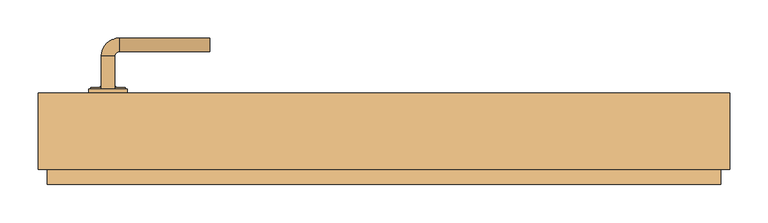
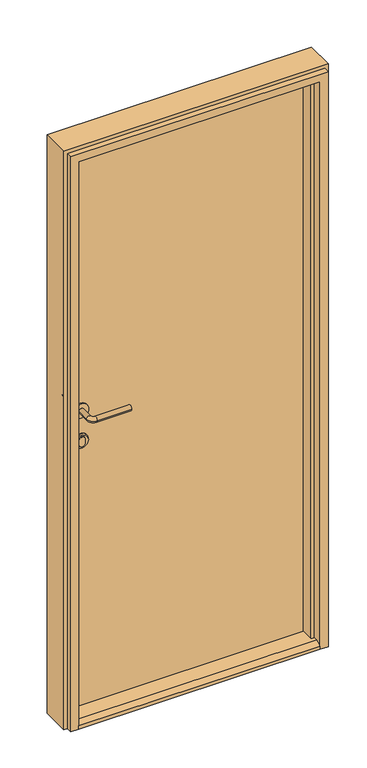
"""IFC4 building model written with IfcOpenShell, lengths in millimetres: door geometry, jeld-wen_interior_door_Stable_GW_single_1.0 : 886 x 2089 mm - M9 x M21."""

import ifcopenshell
import ifcopenshell.guid

model = None  # the IFC model being written
_history = None  # IfcOwnerHistory: only IFC2X3 demands one
_inside = {}  # id of a spatial element -> (the spatial element, [elements in it])
_under = {}  # id of a project, library or spatial element -> (it, [spatial elements below it])
_declared = {}  # id of a project -> (the project, [libraries it declares])
_typed = {}  # id of a type object -> (the type object, [elements of that type])
_made_of = {}  # id of a material, layer set ... -> (it, [elements and type objects made of it])


def new_model(schema):
    """Start an empty IFC model of exactly this schema.

    Asked for "IFC4X3", IfcOpenShell would pick the latest addendum, in which some entities
    have other attributes; the version numbers below select the first issue.
    IFC2X3 requires an IfcOwnerHistory on every rooted entity: one is made here for all.
    """
    global model, _history
    if schema == "IFC4X3":
        model = ifcopenshell.file(schema_version=(4, 3, 0, 0))
    else:
        model = ifcopenshell.file(schema=schema)
    _inside.clear()
    _under.clear()
    _declared.clear()
    _typed.clear()
    _made_of.clear()
    _history = None
    if model.schema == "IFC2X3":
        org = make("IfcOrganization", Name="unknown")
        user = make(
            "IfcPersonAndOrganization",
            ThePerson=make("IfcPerson", FamilyName="unknown"),
            TheOrganization=org,
        )
        app = make(
            "IfcApplication",
            ApplicationDeveloper=org,
            Version="unknown",
            ApplicationFullName="unknown",
            ApplicationIdentifier="unknown",
        )
        _history = make(
            "IfcOwnerHistory",
            OwningUser=user,
            OwningApplication=app,
            ChangeAction="ADDED",
            CreationDate=0,
        )
    return model


def make(cls, **values):
    """One entity of the class cls with the attributes given. An attribute that is None is left unset."""
    return model.create_entity(
        cls, **{name: value for name, value in values.items() if value is not None}
    )


def rooted(cls, **values):
    """An entity with a GlobalId (a new one), such as an element, a storey or a relation."""
    return make(cls, GlobalId=ifcopenshell.guid.new(), OwnerHistory=_history, **values)


def si_unit(unit_type, name, prefix=None):
    """IfcSIUnit, for example si_unit("LENGTHUNIT", "METRE", prefix="MILLI")."""
    return make("IfcSIUnit", UnitType=unit_type, Prefix=prefix, Name=name)


def assignment(units):
    """IfcUnitAssignment: the units of a project."""
    return None if units is None else make("IfcUnitAssignment", Units=units)


def point(xyz):
    """IfcCartesianPoint."""
    return None if xyz is None else make("IfcCartesianPoint", Coordinates=xyz)


def direction(xyz):
    """IfcDirection."""
    return None if xyz is None else make("IfcDirection", DirectionRatios=xyz)


def frame(location, z_axis=None, x_axis=None):
    """IfcAxis2Placement3D, a coordinate frame: its origin and axes. An axis left out is left unset."""
    return make(
        "IfcAxis2Placement3D",
        Location=point(location),
        Axis=direction(z_axis),
        RefDirection=direction(x_axis),
    )


def origin():
    """The frame at (0, 0, 0) with its axes left unset."""
    return frame((0.0, 0.0, 0.0))


def place(relative_to, where):
    """IfcLocalPlacement: puts the frame where relative to a parent placement (None: the world)."""
    return make(
        "IfcLocalPlacement", PlacementRelTo=relative_to, RelativePlacement=where
    )


def context(
    kind, dimensions, precision=None, world=None, true_north=None, identifier=None
):
    """IfcGeometricRepresentationContext, for example the 3D "Model" context."""
    return make(
        "IfcGeometricRepresentationContext",
        ContextIdentifier=identifier,
        ContextType=kind,
        CoordinateSpaceDimension=dimensions,
        Precision=precision,
        WorldCoordinateSystem=world,
        TrueNorth=true_north,
    )


def project(units=None, contexts=None):
    """IfcProject with its units and contexts."""
    return rooted(
        "IfcProject",
        Name="project",
        RepresentationContexts=contexts,
        UnitsInContext=assignment(units),
    )


def spatial(cls, under=None, at=None, **own):
    """A site, building, storey or space (cls), placed at a placement, below another one or the project."""
    s = rooted(cls, ObjectPlacement=at, **own)
    if under is not None:
        _under.setdefault(under.id(), (under, []))[1].append(s)
    return s


def polyline(points):
    """IfcPolyline through the points."""
    return make("IfcPolyline", Points=[point(p) for p in points])


def circle_curve(where, radius):
    """IfcCircle in the frame where."""
    return make("IfcCircle", Position=where, Radius=radius)


def ellipse_curve(where, semi_axis1, semi_axis2):
    """IfcEllipse in the frame where."""
    return make(
        "IfcEllipse", Position=where, SemiAxis1=semi_axis1, SemiAxis2=semi_axis2
    )


def trimmed(basis, trim1, trim2, sense, master):
    """IfcTrimmedCurve: the piece of a basis curve between two trims."""
    return make(
        "IfcTrimmedCurve",
        BasisCurve=basis,
        Trim1=trim1,
        Trim2=trim2,
        SenseAgreement=sense,
        MasterRepresentation=master,
    )


def outline(outer, holes=None, kind="AREA"):
    """IfcArbitraryClosedProfileDef: a profile drawn as a closed curve; with holes, ...WithVoids."""
    if holes is None:
        return make("IfcArbitraryClosedProfileDef", ProfileType=kind, OuterCurve=outer)
    return make(
        "IfcArbitraryProfileDefWithVoids",
        ProfileType=kind,
        OuterCurve=outer,
        InnerCurves=holes,
    )


def extrude(swept, where, along, depth):
    """IfcExtrudedAreaSolid: the profile swept, set in the frame where, extruded along a direction by depth."""
    return make(
        "IfcExtrudedAreaSolid",
        SweptArea=swept,
        Position=where,
        ExtrudedDirection=direction(along),
        Depth=depth,
    )


def faces_of(points, faces, orient=None, outer=None):
    """IfcFace entities. A face is a list of loops; a loop is a list of indices into points, from 0.

    orient and outer hold one flag for each loop. By default every Orientation is true, the
    first loop of a face is its IfcFaceOuterBound and the others are IfcFaceBound.
    """
    made = []
    for i, loops in enumerate(faces):
        bounds = []
        for j, loop in enumerate(loops):
            is_outer = j == 0 if outer is None else outer[i][j]
            bounds.append(
                make(
                    "IfcFaceOuterBound" if is_outer else "IfcFaceBound",
                    Bound=make("IfcPolyLoop", Polygon=[points[k] for k in loop]),
                    Orientation=True if orient is None else orient[i][j],
                )
            )
        made.append(make("IfcFace", Bounds=bounds))
    return made


def faceted_brep(points, faces, orient=None, outer=None, voids=None):
    """IfcFacetedBrep: a solid bounded by flat faces; with voids (closed shells), ...WithVoids."""
    shared = [point(p) for p in points]
    hull = make("IfcClosedShell", CfsFaces=faces_of(shared, faces, orient, outer))
    if voids is None:
        return make("IfcFacetedBrep", Outer=hull)
    return make(
        "IfcFacetedBrepWithVoids",
        Outer=hull,
        Voids=[
            make(cls, CfsFaces=faces_of(shared, fs, o, b)) for cls, fs, o, b in voids
        ],
    )


def shape(context_of_items, identifier, shape_type, items):
    """IfcShapeRepresentation: the items that make up one representation, for example the "Body"."""
    return make(
        "IfcShapeRepresentation",
        ContextOfItems=context_of_items,
        RepresentationIdentifier=identifier,
        RepresentationType=shape_type,
        Items=items,
    )


def source(mapping_origin, context_of_items, identifier, shape_type, items):
    """IfcRepresentationMap: a shape defined once, which mapped items show again and again."""
    return make(
        "IfcRepresentationMap",
        MappingOrigin=mapping_origin,
        MappedRepresentation=shape(context_of_items, identifier, shape_type, items),
    )


def transform(
    local_origin,
    x_axis=None,
    y_axis=None,
    z_axis=None,
    scale=None,
    scale2=None,
    scale3=None,
    uniform=True,
):
    """IfcCartesianTransformationOperator3D, or its non-uniform kind. x_axis, y_axis, z_axis: its Axis1, 2, 3."""
    if uniform:
        return make(
            "IfcCartesianTransformationOperator3D",
            Axis1=direction(x_axis),
            Axis2=direction(y_axis),
            LocalOrigin=point(local_origin),
            Scale=scale,
            Axis3=direction(z_axis),
        )
    return make(
        "IfcCartesianTransformationOperator3DnonUniform",
        Axis1=direction(x_axis),
        Axis2=direction(y_axis),
        LocalOrigin=point(local_origin),
        Scale=scale,
        Axis3=direction(z_axis),
        Scale2=scale2,
        Scale3=scale3,
    )


def mapped(mapping_source, mapping_target):
    """IfcMappedItem: shows the shape of a source again, moved by a transform."""
    return make(
        "IfcMappedItem", MappingSource=mapping_source, MappingTarget=mapping_target
    )


def made_of(thing, what):
    """Note that an element or type object is made of a material, layer set ...; save() writes the relation."""
    if what is not None:
        _made_of.setdefault(what.id(), (what, []))[1].append(thing)
    return thing


def element(
    cls,
    number,
    at=None,
    inside=None,
    cuts=None,
    type_object=None,
    material=None,
    context=None,
    identifier="Body",
    shape_type=None,
    held_by="IfcProductDefinitionShape",
    body=None,
    shapes=None,
    **own,
):
    """One element of the class cls, such as IfcWall. Its Tag is "e" and its number.

    at: its placement. inside: the storey or other place that contains it. cuts: it is an
    opening in that element (IfcRelVoidsElement). A single representation is given by context,
    identifier, shape_type and body (its items); several are given by shapes. held_by: the class
    of the entity that holds the representations. save() writes the other relations.
    """
    e = rooted(cls, Tag="e%d" % number, ObjectPlacement=at, **own)
    if body is not None:
        shapes = [shape(context, identifier, shape_type, body)]
    if shapes is not None:
        e.Representation = make(held_by, Representations=shapes)
    if inside is not None:
        _inside.setdefault(inside.id(), (inside, []))[1].append(e)
    if cuts is not None:
        rooted(
            "IfcRelVoidsElement", RelatingBuildingElement=cuts, RelatedOpeningElement=e
        )
    if type_object is not None:
        _typed.setdefault(type_object.id(), (type_object, []))[1].append(e)
    return made_of(e, material)


def aggregate(whole, parts):
    """IfcRelAggregates: a whole, such as a stair, and the parts it consists of."""
    return rooted("IfcRelAggregates", RelatingObject=whole, RelatedObjects=parts)


def save(model, path):
    """Write the relations noted so far, then the file.

    IfcRelAggregates (storeys below a building ...), IfcRelContainedInSpatialStructure (elements
    in a storey), IfcRelDefinesByType, IfcRelAssociatesMaterial and IfcRelDeclares: one each for
    every whole, place, type object, material and project.
    """
    for whole, parts in _under.values():
        aggregate(whole, parts)
    for where, things in _inside.values():
        rooted(
            "IfcRelContainedInSpatialStructure",
            RelatedElements=things,
            RelatingStructure=where,
        )
    for kind, things in _typed.values():
        rooted("IfcRelDefinesByType", RelatedObjects=things, RelatingType=kind)
    for what, things in _made_of.values():
        rooted("IfcRelAssociatesMaterial", RelatedObjects=things, RelatingMaterial=what)
    for by, libraries in _declared.values():
        rooted("IfcRelDeclares", RelatingContext=by, RelatedDefinitions=libraries)
    model.write(path)


def plane_surface(at):
    """IfcPlane: the flat surface through the origin of the frame at, square to its z axis."""
    return make("IfcPlane", Position=at)


def cylinder_surface(at, radius):
    """IfcCylindricalSurface: all points at the distance radius from the z axis of the frame at."""
    return make("IfcCylindricalSurface", Position=at, Radius=radius)


def revolved_surface(curve, axis_point, axis_direction):
    """IfcSurfaceOfRevolution: the curve turned about the line through axis_point along axis_direction."""
    return make(
        "IfcSurfaceOfRevolution",
        SweptCurve=make("IfcArbitraryOpenProfileDef", ProfileType="CURVE", Curve=curve),
        AxisPosition=make("IfcAxis1Placement", Location=point(axis_point), Axis=direction(axis_direction)),
    )


def advanced_brep(points, edges, surfaces, faces):
    """IfcAdvancedBrep: a solid bounded by faces that lie on surfaces and meet in shared edges.

    An edge is (start, end): straight between two places in points (the first is 0);
    or (start, end, curve); or (start, end, curve, False) where it runs against its curve.
    A face is (place in surfaces, loops), or (place, loops, False) where it looks against
    its surface's normal. A loop lists edges by number (the first is 1), with a minus sign
    where the edge is run from its end to its start. The first loop is the outer one.
    """
    corners = [point(p) for p in points]
    vertices = [make("IfcVertexPoint", VertexGeometry=c) for c in corners]
    made = []
    for start, end, *more in edges:
        made.append(
            make(
                "IfcEdgeCurve",
                EdgeStart=vertices[start],
                EdgeEnd=vertices[end],
                EdgeGeometry=more[0] if more else make("IfcPolyline", Points=[corners[start], corners[end]]),
                SameSense=more[1] if len(more) > 1 else True,
            )
        )
    hull = []
    for where, loops, *sense in faces:
        bounds = []
        for j, loop in enumerate(loops):
            ring = [make("IfcOrientedEdge", EdgeElement=made[abs(k) - 1], Orientation=k > 0) for k in loop]
            bounds.append(
                make(
                    "IfcFaceOuterBound" if j == 0 else "IfcFaceBound",
                    Bound=make("IfcEdgeLoop", EdgeList=ring),
                    Orientation=True,
                )
            )
        hull.append(make("IfcAdvancedFace", Bounds=bounds, FaceSurface=surfaces[where], SameSense=sense[0] if sense else True))
    return make("IfcAdvancedBrep", Outer=make("IfcClosedShell", CfsFaces=hull))


def door_ee319b5f(model_context):
    return source(origin(), model_context, "Body", "SolidModel", [
        advanced_brep(
        [(-385.4704625, 2.0, 983.0), (-340.4704625, 2.0, 983.0), (-371.7998782, 2.0, 995.5684608), (-363.4704625, 2.0, 1000.5), (-362.4704625, 2.0, 1000.5), (-352.9704625, 2.0, 991.0), (-352.9704625, 2.0, 975.0), (-362.4704625, 2.0, 965.5), (-363.4704625, 2.0, 965.5), (-372.9704625, 2.0, 975.0), (-372.9704625, 2.0, 991.0), (-387.9704625, 8.0, 983.0), (-337.9704625, 8.0, 983.0), (-387.9704625, 10.0, 983.0), (-337.9704625, 10.0, 983.0), (-363.4704625, 1.0, 1000.5), (-371.7998782, 1.0, 995.5684608), (-372.9704625, 1.0, 991.0), (-372.9704625, 1.0, 975.0), (-363.4704625, 1.0, 965.5), (-362.4704625, 1.0, 965.5), (-352.9704625, 1.0, 975.0), (-352.9704625, 1.0, 991.0), (-362.4704625, 1.0, 1000.5)],
        [
            (0, 1, circle_curve(frame((-362.9704625, 2.0, 983.0), z_axis=(0.0, -1.0, 0.0), x_axis=(-1.0, 0.0, 0.0)), 22.5)),
            (1, 0, circle_curve(frame((-362.9704625, 2.0, 983.0), z_axis=(0.0, -1.0, 0.0), x_axis=(1.0, 0.0, 0.0)), 22.5)),
            (2, 3, circle_curve(frame((-363.4704625, 2.0, 991.0), z_axis=(0.0, 1.0, 0.0), x_axis=(-1.0, 0.0, 0.0)), 9.5)),
            (3, 4),
            (4, 5, circle_curve(frame((-362.4704625, 2.0, 991.0), z_axis=(0.0, 1.0, 0.0), x_axis=(-1.0, 0.0, 0.0)), 9.5)),
            (5, 6),
            (6, 7, circle_curve(frame((-362.4704625, 2.0, 975.0), z_axis=(0.0, 1.0, 0.0), x_axis=(-1.0, 0.0, 0.0)), 9.5)),
            (7, 8),
            (8, 9, circle_curve(frame((-363.4704625, 2.0, 975.0), z_axis=(0.0, 1.0, 0.0), x_axis=(-1.0, 0.0, 0.0)), 9.5)),
            (9, 10),
            (10, 2, circle_curve(frame((-363.4704625, 2.0, 991.0), z_axis=(0.0, 1.0, 0.0), x_axis=(-1.0, 0.0, 0.0)), 9.5)),
            (0, 11),
            (11, 12, circle_curve(frame((-362.9704625, 8.0, 983.0), z_axis=(0.0, -1.0, 0.0), x_axis=(-1.0, 0.0, 0.0)), 25.0)),
            (12, 1),
            (12, 11, circle_curve(frame((-362.9704625, 8.0, 983.0), z_axis=(0.0, -1.0, 0.0), x_axis=(1.0, 0.0, 0.0)), 25.0)),
            (13, 14, circle_curve(frame((-362.9704625, 10.0, 983.0), z_axis=(0.0, 1.0, 0.0), x_axis=(1.0, 0.0, 0.0)), 25.0)),
            (14, 13, circle_curve(frame((-362.9704625, 10.0, 983.0), z_axis=(0.0, 1.0, 0.0), x_axis=(1.0, 0.0, 0.0)), 25.0)),
            (14, 12),
            (11, 13),
            (15, 16, circle_curve(frame((-363.4704625, 1.0, 991.0), z_axis=(0.0, -1.0, 0.0), x_axis=(-1.0, 0.0, 0.0)), 9.5)),
            (16, 17, circle_curve(frame((-363.4704625, 1.0, 991.0), z_axis=(0.0, -1.0, 0.0), x_axis=(-1.0, 0.0, 0.0)), 9.5)),
            (17, 18),
            (18, 19, circle_curve(frame((-363.4704625, 1.0, 975.0), z_axis=(0.0, -1.0, 0.0), x_axis=(-1.0, 0.0, 0.0)), 9.5)),
            (19, 20),
            (20, 21, circle_curve(frame((-362.4704625, 1.0, 975.0), z_axis=(0.0, -1.0, 0.0), x_axis=(-1.0, 0.0, 0.0)), 9.5)),
            (21, 22),
            (22, 23, circle_curve(frame((-362.4704625, 1.0, 991.0), z_axis=(0.0, -1.0, 0.0), x_axis=(-1.0, 0.0, 0.0)), 9.5)),
            (23, 15),
            (15, 3),
            (2, 16),
            (10, 17),
            (9, 18),
            (8, 19),
            (7, 20),
            (6, 21),
            (5, 22),
            (4, 23),
        ],
        [
            plane_surface(frame((-362.9704625, 2.0, 983.0), z_axis=(0.0, -1.0, 0.0), x_axis=(0.0, 0.0, -1.0))),
            revolved_surface(polyline([(-385.4704625, 2.0, 983.0), (-387.9704625, 8.0, 983.0)]), (-362.9704625, -52.0, 983.0), (0.0, 1.0, 0.0)),
            revolved_surface(polyline([(-340.4704625, 2.0, 983.0), (-337.9704625, 8.0, 983.0)]), (-362.9704625, -52.0, 983.0), (0.0, 1.0, 0.0)),
            plane_surface(frame((-337.9704625, 10.0, 983.0), z_axis=(0.0, 1.0, 0.0), x_axis=(0.0, 0.0, -1.0))),
            cylinder_surface(frame((-362.9704625, 10.0, 983.0), z_axis=(0.0, -1.0, 0.0), x_axis=(1.0, 0.0, 0.0)), 25.0),
            plane_surface(frame((-372.9704625, 1.0, 991.0), z_axis=(0.0, -1.0, 0.0), x_axis=(0.0, 0.0, -1.0))),
            cylinder_surface(frame((-363.4704625, 2.0, 991.0), z_axis=(0.0, -1.0, 0.0), x_axis=(-1.0, 0.0, 0.0)), 9.5),
            plane_surface(frame((-372.9704625, 1.0, 991.0), z_axis=(-1.0, 0.0, 0.0), x_axis=(0.0, 1.0, 0.0))),
            cylinder_surface(frame((-363.4704625, 2.0, 975.0), z_axis=(0.0, -1.0, 0.0), x_axis=(-1.0, 0.0, 0.0)), 9.5),
            plane_surface(frame((-363.4704625, 1.0, 965.5), z_axis=(0.0, 0.0, -1.0), x_axis=(0.0, 1.0, 0.0))),
            cylinder_surface(frame((-362.4704625, 2.0, 975.0), z_axis=(0.0, -1.0, 0.0), x_axis=(-1.0, 0.0, 0.0)), 9.5),
            plane_surface(frame((-352.9704625, 1.0, 975.0), z_axis=(1.0, 0.0, 0.0), x_axis=(0.0, 1.0, 0.0))),
            cylinder_surface(frame((-362.4704625, 2.0, 991.0), z_axis=(0.0, -1.0, 0.0), x_axis=(-1.0, 0.0, 0.0)), 9.5),
            plane_surface(frame((-362.4704625, 1.0, 1000.5), z_axis=(0.0, 0.0, 1.0), x_axis=(0.0, 1.0, 0.0))),
        ],
        [
            (0, [[1, 2], [3, 4, 5, 6, 7, 8, 9, 10, 11]]),
            (1, [[-1, 12, 13, 14]]),
            (2, [[-2, -14, 15, -12]]),
            (3, [[16, 17]]),
            (4, [[-17, 18, -13, 19]]),
            (4, [[-16, -19, -15, -18]]),
            (5, [[20, 21, 22, 23, 24, 25, 26, 27, 28]]),
            (6, [[-20, 29, -3, 30]]),
            (6, [[-21, -30, -11, 31]]),
            (7, [[-22, -31, -10, 32]]),
            (8, [[-23, -32, -9, 33]]),
            (9, [[-24, -33, -8, 34]]),
            (10, [[-25, -34, -7, 35]]),
            (11, [[-26, -35, -6, 36]]),
            (12, [[-27, -36, -5, 37]]),
            (13, [[-28, -37, -4, -29]]),
        ],
    ),
        advanced_brep(
        [(-385.4704625, 58.0, 983.0), (-340.4704625, 58.0, 983.0), (-371.7998782, 58.0, 995.5684608), (-372.9704625, 58.0, 991.0), (-372.9704625, 58.0, 975.0), (-363.4704625, 58.0, 965.5), (-362.4704625, 58.0, 965.5), (-352.9704625, 58.0, 975.0), (-352.9704625, 58.0, 991.0), (-362.4704625, 58.0, 1000.5), (-363.4704625, 58.0, 1000.5), (-337.9704625, 52.0, 983.0), (-387.9704625, 52.0, 983.0), (-387.9704625, 50.0, 983.0), (-337.9704625, 50.0, 983.0), (-363.4704625, 59.0, 1000.5), (-362.4704625, 59.0, 1000.5), (-352.9704625, 59.0, 991.0), (-352.9704625, 59.0, 975.0), (-362.4704625, 59.0, 965.5), (-363.4704625, 59.0, 965.5), (-372.9704625, 59.0, 975.0), (-372.9704625, 59.0, 991.0), (-371.7998782, 59.0, 995.5684608)],
        [
            (0, 1, circle_curve(frame((-362.9704625, 58.0, 983.0), z_axis=(0.0, 1.0, 0.0), x_axis=(1.0, 0.0, 0.0)), 22.5)),
            (1, 0, circle_curve(frame((-362.9704625, 58.0, 983.0), z_axis=(0.0, 1.0, 0.0), x_axis=(-1.0, 0.0, 0.0)), 22.5)),
            (2, 3, circle_curve(frame((-363.4704625, 58.0, 991.0), z_axis=(0.0, -1.0, 0.0), x_axis=(-1.0, 0.0, 0.0)), 9.5)),
            (3, 4),
            (4, 5, circle_curve(frame((-363.4704625, 58.0, 975.0), z_axis=(0.0, -1.0, 0.0), x_axis=(-1.0, 0.0, 0.0)), 9.5)),
            (5, 6),
            (6, 7, circle_curve(frame((-362.4704625, 58.0, 975.0), z_axis=(0.0, -1.0, 0.0), x_axis=(-1.0, 0.0, 0.0)), 9.5)),
            (7, 8),
            (8, 9, circle_curve(frame((-362.4704625, 58.0, 991.0), z_axis=(0.0, -1.0, 0.0), x_axis=(-1.0, 0.0, 0.0)), 9.5)),
            (9, 10),
            (10, 2, circle_curve(frame((-363.4704625, 58.0, 991.0), z_axis=(0.0, -1.0, 0.0), x_axis=(-1.0, 0.0, 0.0)), 9.5)),
            (1, 11),
            (11, 12, circle_curve(frame((-362.9704625, 52.0, 983.0), z_axis=(0.0, 1.0, 0.0), x_axis=(-1.0, 0.0, 0.0)), 25.0)),
            (12, 0),
            (12, 11, circle_curve(frame((-362.9704625, 52.0, 983.0), z_axis=(0.0, 1.0, 0.0), x_axis=(1.0, 0.0, 0.0)), 25.0)),
            (13, 14, circle_curve(frame((-362.9704625, 50.0, 983.0), z_axis=(0.0, -1.0, 0.0), x_axis=(1.0, 0.0, 0.0)), 25.0)),
            (14, 13, circle_curve(frame((-362.9704625, 50.0, 983.0), z_axis=(0.0, -1.0, 0.0), x_axis=(1.0, 0.0, 0.0)), 25.0)),
            (13, 12),
            (11, 14),
            (15, 16),
            (16, 17, circle_curve(frame((-362.4704625, 59.0, 991.0), z_axis=(0.0, 1.0, 0.0), x_axis=(-1.0, 0.0, 0.0)), 9.5)),
            (17, 18),
            (18, 19, circle_curve(frame((-362.4704625, 59.0, 975.0), z_axis=(0.0, 1.0, 0.0), x_axis=(-1.0, 0.0, 0.0)), 9.5)),
            (19, 20),
            (20, 21, circle_curve(frame((-363.4704625, 59.0, 975.0), z_axis=(0.0, 1.0, 0.0), x_axis=(-1.0, 0.0, 0.0)), 9.5)),
            (21, 22),
            (22, 23, circle_curve(frame((-363.4704625, 59.0, 991.0), z_axis=(0.0, 1.0, 0.0), x_axis=(-1.0, 0.0, 0.0)), 9.5)),
            (23, 15, circle_curve(frame((-363.4704625, 59.0, 991.0), z_axis=(0.0, 1.0, 0.0), x_axis=(-1.0, 0.0, 0.0)), 9.5)),
            (23, 2),
            (10, 15),
            (22, 3),
            (21, 4),
            (20, 5),
            (19, 6),
            (18, 7),
            (17, 8),
            (16, 9),
        ],
        [
            plane_surface(frame((-362.9704625, 58.0, 983.0), z_axis=(0.0, 1.0, 0.0), x_axis=(0.0, 0.0, -1.0))),
            revolved_surface(polyline([(-340.4704625, 58.0, 983.0), (-337.9704625, 52.0, 983.0)]), (-362.9704625, 112.0, 983.0), (0.0, -1.0, 0.0)),
            revolved_surface(polyline([(-385.4704625, 58.0, 983.0), (-387.9704625, 52.0, 983.0)]), (-362.9704625, 112.0, 983.0), (0.0, -1.0, 0.0)),
            plane_surface(frame((-337.9704625, 50.0, 983.0), z_axis=(0.0, -1.0, 0.0), x_axis=(0.0, 0.0, -1.0))),
            cylinder_surface(frame((-362.9704625, 50.0, 983.0), z_axis=(0.0, 1.0, 0.0), x_axis=(1.0, 0.0, 0.0)), 25.0),
            plane_surface(frame((-372.9704625, 59.0, 991.0), z_axis=(0.0, 1.0, 0.0), x_axis=(0.0, 0.0, -1.0))),
            cylinder_surface(frame((-363.4704625, 58.0, 991.0), z_axis=(0.0, 1.0, 0.0), x_axis=(-1.0, 0.0, 0.0)), 9.5),
            plane_surface(frame((-372.9704625, 59.0, 991.0), z_axis=(-1.0, 0.0, 0.0), x_axis=(0.0, -1.0, 0.0))),
            cylinder_surface(frame((-363.4704625, 58.0, 975.0), z_axis=(0.0, 1.0, 0.0), x_axis=(-1.0, 0.0, 0.0)), 9.5),
            plane_surface(frame((-363.4704625, 59.0, 965.5), z_axis=(0.0, 0.0, -1.0), x_axis=(0.0, -1.0, 0.0))),
            cylinder_surface(frame((-362.4704625, 58.0, 975.0), z_axis=(0.0, 1.0, 0.0), x_axis=(-1.0, 0.0, 0.0)), 9.5),
            plane_surface(frame((-352.9704625, 59.0, 975.0), z_axis=(1.0, 0.0, 0.0), x_axis=(0.0, -1.0, 0.0))),
            cylinder_surface(frame((-362.4704625, 58.0, 991.0), z_axis=(0.0, 1.0, 0.0), x_axis=(-1.0, 0.0, 0.0)), 9.5),
            plane_surface(frame((-362.4704625, 59.0, 1000.5), z_axis=(0.0, 0.0, 1.0), x_axis=(0.0, -1.0, 0.0))),
        ],
        [
            (0, [[1, 2], [3, 4, 5, 6, 7, 8, 9, 10, 11]]),
            (1, [[12, 13, 14, -2]]),
            (2, [[-14, 15, -12, -1]]),
            (3, [[16, 17]]),
            (4, [[18, -13, 19, -16]]),
            (4, [[-19, -15, -18, -17]]),
            (5, [[20, 21, 22, 23, 24, 25, 26, 27, 28]]),
            (6, [[29, -11, 30, -28]]),
            (6, [[31, -3, -29, -27]]),
            (7, [[32, -4, -31, -26]]),
            (8, [[33, -5, -32, -25]]),
            (9, [[34, -6, -33, -24]]),
            (10, [[35, -7, -34, -23]]),
            (11, [[36, -8, -35, -22]]),
            (12, [[37, -9, -36, -21]]),
            (13, [[-30, -10, -37, -20]]),
        ],
    ),
        advanced_brep(
        [(-387.9704625, 4.0, 1093.0), (-337.9704625, 4.0, 1093.0), (-354.0050698, 4.0, 1093.0), (-371.9358552, 4.0, 1093.0), (-387.9704625, 10.0, 1093.0), (-337.9704625, 10.0, 1093.0), (-371.9358552, -38.9627146, 1093.0), (-354.0050698, -38.9627146, 1093.0), (-347.9704625, -62.9281073, 1093.0), (-347.9704625, -44.9973219, 1093.0), (-228.9704625, -44.9973219, 1093.0), (-228.9704625, -62.9281073, 1093.0)],
        [
            (0, 1, circle_curve(frame((-362.9704625, 4.0, 1093.0), z_axis=(0.0, -1.0, 0.0), x_axis=(1.0, 0.0, 0.0)), 25.0)),
            (1, 0, circle_curve(frame((-362.9704625, 4.0, 1093.0), z_axis=(0.0, -1.0, 0.0), x_axis=(1.0, 0.0, 0.0)), 25.0)),
            (2, 3, circle_curve(frame((-362.9704625, 4.0, 1093.0), z_axis=(0.0, 1.0, 0.0), x_axis=(-1.0, 0.0, 0.0)), 8.9653927)),
            (3, 2, circle_curve(frame((-362.9704625, 4.0, 1093.0), z_axis=(0.0, 1.0, 0.0), x_axis=(-1.0, 0.0, 0.0)), 8.9653927)),
            (4, 5, circle_curve(frame((-362.9704625, 10.0, 1093.0), z_axis=(0.0, 1.0, 0.0), x_axis=(1.0, 0.0, 0.0)), 25.0)),
            (5, 4, circle_curve(frame((-362.9704625, 10.0, 1093.0), z_axis=(0.0, 1.0, 0.0), x_axis=(1.0, 0.0, 0.0)), 25.0)),
            (0, 4),
            (5, 1),
            (3, 6),
            (6, 7, circle_curve(frame((-362.9704625, -38.9627146, 1093.0), z_axis=(0.0, 1.0, 0.0), x_axis=(-1.0, 0.0, 0.0)), 8.9653927)),
            (7, 2),
            (7, 6, circle_curve(frame((-362.9704625, -38.9627146, 1093.0), z_axis=(0.0, 1.0, 0.0), x_axis=(-1.0, 0.0, 0.0)), 8.9653927)),
            (6, 8, circle_curve(frame((-347.9704625, -38.9627146, 1093.0), z_axis=(0.0, 0.0, 1.0), x_axis=(-1.0, 0.0, 0.0)), 23.9653927)),
            (8, 9, circle_curve(frame((-347.9704625, -53.9627146, 1093.0), z_axis=(-1.0, 0.0, 0.0), x_axis=(0.0, -1.0, 0.0)), 8.9653927)),
            (9, 7, circle_curve(frame((-347.9704625, -38.9627146, 1093.0), z_axis=(0.0, 0.0, -1.0), x_axis=(-1.0, 0.0, 0.0)), 6.0346073)),
            (9, 8, circle_curve(frame((-347.9704625, -53.9627146, 1093.0), z_axis=(-1.0, 0.0, 0.0), x_axis=(0.0, -1.0, 0.0)), 8.9653927)),
            (10, 11, circle_curve(frame((-228.9704625, -53.9627146, 1093.0), z_axis=(1.0, 0.0, 0.0), x_axis=(0.0, -1.0, 0.0)), 8.9653927)),
            (11, 10, circle_curve(frame((-228.9704625, -53.9627146, 1093.0), z_axis=(1.0, 0.0, 0.0), x_axis=(0.0, -1.0, 0.0)), 8.9653927)),
            (8, 11),
            (10, 9),
        ],
        [
            plane_surface(frame((-337.9704625, 4.0, 1093.0), z_axis=(0.0, -1.0, 0.0), x_axis=(0.0, 0.0, -1.0))),
            plane_surface(frame((-337.9704625, 10.0, 1093.0), z_axis=(0.0, 1.0, 0.0), x_axis=(0.0, 0.0, 1.0))),
            cylinder_surface(frame((-362.9704625, 4.0, 1093.0), z_axis=(0.0, 1.0, 0.0), x_axis=(1.0, 0.0, 0.0)), 25.0),
            cylinder_surface(frame((-362.9704625, 4.0, 1093.0), z_axis=(0.0, 1.0, 0.0), x_axis=(-1.0, 0.0, 0.0)), 8.9653927),
            revolved_surface(trimmed(ellipse_curve(frame((-362.9704625, -38.9627146, 1093.0), z_axis=(0.0, -1.0, 0.0), x_axis=(-1.0, 0.0, 0.0)), 8.9653927, 8.9653927), [point((-354.0050698, -38.9627146, 1093.0))], [point((-371.9358552, -38.9627146, 1093.0))], True, "CARTESIAN"), (-347.9704625, -38.9627146, 1093.0), (0.0, 0.0, -1.0)),
            revolved_surface(trimmed(ellipse_curve(frame((-362.9704625, -38.9627146, 1093.0), z_axis=(0.0, -1.0, 0.0), x_axis=(-1.0, 0.0, 0.0)), 8.9653927, 8.9653927), [point((-371.9358552, -38.9627146, 1093.0))], [point((-354.0050698, -38.9627146, 1093.0))], True, "CARTESIAN"), (-347.9704625, -38.9627146, 1093.0), (0.0, 0.0, -1.0)),
            plane_surface(frame((-228.9704625, -53.9627146, 1093.0), z_axis=(1.0, 0.0, 0.0), x_axis=(0.0, 0.0, 1.0))),
            cylinder_surface(frame((-347.9704625, -53.9627146, 1093.0), z_axis=(-1.0, 0.0, 0.0), x_axis=(0.0, -1.0, 0.0)), 8.9653927),
        ],
        [
            (0, [[1, 2], [3, 4]]),
            (1, [[5, 6]]),
            (2, [[7, -6, 8, -1]]),
            (2, [[-8, -5, -7, -2]]),
            (3, [[-4, 9, 10, 11]]),
            (3, [[12, -9, -3, -11]]),
            (4, [[13, 14, 15, -10]]),
            (5, [[-15, 16, -13, -12]]),
            (6, [[17, 18]]),
            (7, [[19, -17, 20, -14]]),
            (7, [[-20, -18, -19, -16]]),
        ],
    ),
        advanced_brep(
        [(-387.9704625, 56.0, 1093.0), (-337.9704625, 56.0, 1093.0), (-354.0050698, 56.0, 1093.0), (-371.9358552, 56.0, 1093.0), (-387.9704625, 50.0, 1093.0), (-337.9704625, 50.0, 1093.0), (-354.0050698, 98.9627146, 1093.0), (-371.9358552, 98.9627146, 1093.0), (-347.9704625, 104.9973219, 1093.0), (-347.9704625, 122.9281073, 1093.0), (-228.9704625, 104.9973219, 1093.0), (-228.9704625, 122.9281073, 1093.0)],
        [
            (0, 1, circle_curve(frame((-362.9704625, 56.0, 1093.0), z_axis=(0.0, 1.0, 0.0), x_axis=(1.0, 0.0, 0.0)), 25.0)),
            (1, 0, circle_curve(frame((-362.9704625, 56.0, 1093.0), z_axis=(0.0, 1.0, 0.0), x_axis=(1.0, 0.0, 0.0)), 25.0)),
            (2, 3, circle_curve(frame((-362.9704625, 56.0, 1093.0), z_axis=(0.0, -1.0, 0.0), x_axis=(-1.0, 0.0, 0.0)), 8.9653927)),
            (3, 2, circle_curve(frame((-362.9704625, 56.0, 1093.0), z_axis=(0.0, -1.0, 0.0), x_axis=(-1.0, 0.0, 0.0)), 8.9653927)),
            (4, 5, circle_curve(frame((-362.9704625, 50.0, 1093.0), z_axis=(0.0, -1.0, 0.0), x_axis=(1.0, 0.0, 0.0)), 25.0)),
            (5, 4, circle_curve(frame((-362.9704625, 50.0, 1093.0), z_axis=(0.0, -1.0, 0.0), x_axis=(1.0, 0.0, 0.0)), 25.0)),
            (1, 5),
            (4, 0),
            (2, 6),
            (6, 7, circle_curve(frame((-362.9704625, 98.9627146, 1093.0), z_axis=(0.0, -1.0, 0.0), x_axis=(-1.0, 0.0, 0.0)), 8.9653927)),
            (7, 3),
            (7, 6, circle_curve(frame((-362.9704625, 98.9627146, 1093.0), z_axis=(0.0, -1.0, 0.0), x_axis=(-1.0, 0.0, 0.0)), 8.9653927)),
            (6, 8, circle_curve(frame((-347.9704625, 98.9627146, 1093.0), z_axis=(0.0, 0.0, -1.0), x_axis=(-1.0, 0.0, 0.0)), 6.0346073)),
            (8, 9, circle_curve(frame((-347.9704625, 113.9627146, 1093.0), z_axis=(-1.0, 0.0, 0.0), x_axis=(0.0, 1.0, 0.0)), 8.9653927)),
            (9, 7, circle_curve(frame((-347.9704625, 98.9627146, 1093.0), z_axis=(0.0, 0.0, 1.0), x_axis=(-1.0, 0.0, 0.0)), 23.9653927)),
            (9, 8, circle_curve(frame((-347.9704625, 113.9627146, 1093.0), z_axis=(-1.0, 0.0, 0.0), x_axis=(0.0, 1.0, 0.0)), 8.9653927)),
            (10, 11, circle_curve(frame((-228.9704625, 113.9627146, 1093.0), z_axis=(1.0, 0.0, 0.0), x_axis=(0.0, 1.0, 0.0)), 8.9653927)),
            (11, 10, circle_curve(frame((-228.9704625, 113.9627146, 1093.0), z_axis=(1.0, 0.0, 0.0), x_axis=(0.0, 1.0, 0.0)), 8.9653927)),
            (8, 10),
            (11, 9),
        ],
        [
            plane_surface(frame((-337.9704625, 56.0, 1093.0), z_axis=(0.0, 1.0, 0.0), x_axis=(0.0, 0.0, -1.0))),
            plane_surface(frame((-337.9704625, 50.0, 1093.0), z_axis=(0.0, -1.0, 0.0), x_axis=(0.0, 0.0, 1.0))),
            cylinder_surface(frame((-362.9704625, 56.0, 1093.0), z_axis=(0.0, -1.0, 0.0), x_axis=(1.0, 0.0, 0.0)), 25.0),
            cylinder_surface(frame((-362.9704625, 56.0, 1093.0), z_axis=(0.0, -1.0, 0.0), x_axis=(-1.0, 0.0, 0.0)), 8.9653927),
            revolved_surface(trimmed(ellipse_curve(frame((-362.9704625, 98.9627146, 1093.0), z_axis=(0.0, -1.0, 0.0), x_axis=(-1.0, 0.0, 0.0)), 8.9653927, 8.9653927), [point((-354.0050698, 98.9627146, 1093.0))], [point((-371.9358552, 98.9627146, 1093.0))], True, "CARTESIAN"), (-347.9704625, 98.9627146, 1093.0), (0.0, 0.0, -1.0)),
            revolved_surface(trimmed(ellipse_curve(frame((-362.9704625, 98.9627146, 1093.0), z_axis=(0.0, -1.0, 0.0), x_axis=(-1.0, 0.0, 0.0)), 8.9653927, 8.9653927), [point((-371.9358552, 98.9627146, 1093.0))], [point((-354.0050698, 98.9627146, 1093.0))], True, "CARTESIAN"), (-347.9704625, 98.9627146, 1093.0), (0.0, 0.0, -1.0)),
            plane_surface(frame((-228.9704625, 113.9627146, 1093.0), z_axis=(1.0, 0.0, 0.0), x_axis=(0.0, 0.0, 1.0))),
            cylinder_surface(frame((-347.9704625, 113.9627146, 1093.0), z_axis=(-1.0, 0.0, 0.0), x_axis=(0.0, 1.0, 0.0)), 8.9653927),
        ],
        [
            (0, [[1, 2], [3, 4]]),
            (1, [[5, 6]]),
            (2, [[-2, 7, -5, 8]]),
            (2, [[-1, -8, -6, -7]]),
            (3, [[9, 10, 11, -3]]),
            (3, [[-9, -4, -11, 12]]),
            (4, [[-10, 13, 14, 15]]),
            (5, [[-12, -15, 16, -13]]),
            (6, [[17, 18]]),
            (7, [[-14, 19, -18, 20]]),
            (7, [[-16, -20, -17, -19]]),
        ],
    ),
        faceted_brep([(415.0, 50.0, 0.0), (415.0, 50.0, 14.0), (415.0, 8.0, 14.0), (415.0, 8.0, 0.0), (415.0, -50.31911, 22.0), (415.0, -70.0, 11.7852546), (415.0, -70.0, 0.0), (415.0, -36.0, 0.0), (415.0, -36.0, 22.0), (-415.0, -70.0, 0.0), (-415.0, -70.0, 11.7852546), (-415.0, -50.31911, 22.0), (-415.0, -36.0, 22.0), (-415.0, -36.0, 0.0), (-415.0, 8.0, 14.0), (-415.0, 50.0, 14.0), (-415.0, 50.0, 0.0), (-415.0, 8.0, 0.0), (-403.0, -36.0, 0.0), (-403.0, 8.0, 0.0), (403.0, 8.0, 0.0), (403.0, -36.0, 0.0), (-403.0, 8.0, 14.0), (403.0, 8.0, 14.0), (-403.0, 8.0, 22.0), (403.0, 8.0, 22.0), (403.0, -36.0, 22.0), (-403.0, -36.0, 22.0)], [[[0, 1, 2, 3]], [[4, 5, 6, 7, 8]], [[9, 10, 11, 12, 13]], [[14, 15, 16, 17]], [[6, 9, 13, 18, 19, 17, 16, 0, 3, 20, 21, 7]], [[1, 0, 16, 15]], [[2, 1, 15, 14, 22, 23]], [[22, 24, 25, 23]], [[11, 4, 8, 26, 25, 24, 27, 12]], [[5, 4, 11, 10]], [[6, 5, 10, 9]], [[19, 22, 14, 17]], [[27, 18, 13, 12]], [[22, 19, 18, 27, 24]], [[23, 20, 3, 2]], [[21, 26, 8, 7]], [[20, 23, 25, 26, 21]]]),
        extrude(outline(polyline([(412.5, 10.0), (-412.5, 10.0), (-412.5, 50.0), (412.5, 50.0), (412.5, 10.0)])), frame((0.0, 0.0, 18.0), z_axis=(0.0, 0.0, 1.0), x_axis=(1.0, 0.0, 0.0)), (0.0, 0.0, 1.0), 2040.0),
        faceted_brep([(443.0, -70.0, 0.0), (415.0, -70.0, 0.0), (415.0, -36.0, 0.0), (403.0, -36.0, 0.0), (403.0, 8.0, 0.0), (415.0, 8.0, 0.0), (415.0, 50.0, 0.0), (443.0, 50.0, 0.0), (443.0, -70.0, 2089.0), (-443.0, -70.0, 2089.0), (-443.0, -70.0, 0.0), (-415.0, -70.0, 0.0), (-415.0, -70.0, 2061.0), (415.0, -70.0, 2061.0), (415.0, -36.0, 2061.0), (-415.0, -36.0, 2061.0), (-415.0, -36.0, 0.0), (-403.0, -36.0, 0.0), (-403.0, -36.0, 2049.0), (403.0, -36.0, 2049.0), (403.0, 8.0, 2049.0), (-403.0, 8.0, 2049.0), (-403.0, 8.0, 0.0), (-415.0, 8.0, 0.0), (-415.0, 8.0, 2061.0), (415.0, 8.0, 2061.0), (415.0, 50.0, 2061.0), (-415.0, 50.0, 2061.0), (-415.0, 50.0, 0.0), (-443.0, 50.0, 0.0), (-443.0, 50.0, 2089.0), (443.0, 50.0, 2089.0)], [[[0, 1, 2, 3, 4, 5, 6, 7]], [[1, 0, 8, 9, 10, 11, 12, 13]], [[2, 1, 13, 14]], [[3, 2, 14, 15, 16, 17, 18, 19]], [[4, 3, 19, 20]], [[5, 4, 20, 21, 22, 23, 24, 25]], [[6, 5, 25, 26]], [[7, 6, 26, 27, 28, 29, 30, 31]], [[0, 7, 31, 8]], [[9, 30, 29, 10]], [[10, 29, 28, 23, 22, 17, 16, 11]], [[15, 12, 11, 16]], [[21, 18, 17, 22]], [[27, 24, 23, 28]], [[14, 13, 12, 15]], [[20, 19, 18, 21]], [[26, 25, 24, 27]], [[8, 31, 30, 9]]]),
        extrude(outline(polyline([(0.0, -455.0), (0.0, -443.0), (2089.0, -443.0), (2089.0, 443.0), (0.0, 443.0), (0.0, 455.0), (2101.0, 455.0), (2101.0, -455.0), (0.0, -455.0)])), frame((0.0, -50.0, 0.0), z_axis=(0.0, 1.0, 0.0), x_axis=(0.0, 0.0, 1.0)), (0.0, 0.0, 1.0), 100.0),
    ])


if __name__ == "__main__":
    model = new_model("IFC4")
    model_context = context("Model", 3, world=origin())
    ifc_project = project(units=[si_unit("LENGTHUNIT", "METRE", prefix="MILLI")], contexts=[model_context])
    site = spatial("IfcSite", under=ifc_project)
    building = spatial("IfcBuilding", under=site)
    placement = place(None, origin())
    door_shape = door_ee319b5f(model_context)
    element("IfcDoor", 1, ObjectType="jeld-wen_interior_door_Stable_GW_single_1.0 : 886 x 2089 mm - M9 x M21", at=placement, inside=building, context=model_context, shape_type="MappedRepresentation", body=[
        mapped(door_shape, transform((0.0, 0.0, 0.0), x_axis=(1.0, 0.0, 0.0), y_axis=(0.0, 1.0, 0.0), z_axis=(0.0, 0.0, 1.0))),
    ])
    save(model, "model.ifc")

# Revit data of these elements
# Type "jeld-wen_interior_door_Stable_GW_single_1.0 : 886 x 2089 mm - M9 x M21"
#   Type Mark = "42"
#   Youtube clip = ""
#   Uniclass 2.0 Description = "Doorsets"
#   Uniclass 2.0 Code = "PR-59-23"
#   Uniclass 1.4 Description = "Doors"
#   Uniclass 1.4 Code = "L411"
#   UNSPSC Code = "301715"
#   Technical description = "http://www.swedoor.se/mattofakta"
#   Region South America = "None"
#   Region Oceania = "None"
#   Region North America = "None"
#   Region Middle East = "None"
#   Region Europe = "DK, FI, IS, NO, SE"
#   Region Asia = "None"
#   Region Antarctica = "None"
#   Region Africa = "None"
#   QR code = "http://bimobject.com/swedoor-jeld-wen/product/int_door_stable_nature"
#   Product group = "ADVANCE-LINE - Stable Nature"
#   Product family = "Interior doors"
#   Product data url = "http://bimobject.com/swedoor-jeld-wen/product/int_door_stable_nature"
#   Product certification = "http://www.swedoor.se/goda-raad/download-center/#59360"
#   Product SKU = "int_door_stable_nature"
#   Product Guid = "2c907816-df84-4119-9f23-2aac3199c8d4"
#   NBS Reference Description = "Doorsets"
#   NBS Reference Code = "59-23"
#   Material secondary = ""
#   Material main = "Wood"
#   Manufacturer name = "SWEDOOR JELD-WEN "
#   Manufacturer country = "Denmark"
#   Manufacturer = "JELD-WEN"
#   Installation instructions = "http://www.swedoor.se/goda-raad/download-center/#6849"
#   IFC Classification = "Door"
#   EAN code = ""
#   Design country = "Denmark"
#   Date of publishing = "2015-06-11"
#   COBIe Type Category = ""
#   BIMobject category = "Doors"
#   Analytic Construction = "<None>"
#   Weight Net (Kg) = 0
#   Rough Width = 910 mm
#   Rough Height = 2101 mm
#   Nominal width = 0
#   Nominal height = 0
#   Frame Projection Ext. = 25 mm
#   Frame Projection Int. = 25 mm
#   Frame Width = 75 mm
#   Height = 2089 mm
#   Width = 886 mm
#   Frame Depth [instance default] = 120 mm
#   Door Panel Width = 825 mm
#   Door Panel Height = 2040 mm
#   Clear Opening 90° [instance default] = 760 mm
#   Standard Threshold 9 mm [instance default] = no
#   Standard Threshold 25 mm [instance default] = no
#   Standard Threshold 22 mm [instance default] = yes
#   Edition number = 1
#   Surface Material [instance default] = element 555374
#   Frame Surface Finish Material = White
#   Door Surface Finish Material = White paint
#   Function = (empty or 0)
#   Wall Closure = (empty or 0)
# Element 1 (IfcDoor, "jeld-wen_interior_door_Stable_GW_single_1.0 : 886 x 2089 mm - M9 x M21")
#   Materials on its faces: "Titanium", "White", "Wood (Oak)", "White paint"
# Materials
#   "White": class "Paint/Coating", colour RGB 250 250 250, transparency 0, Manufacturer = "Modernform", Description = "WH", Cost = 0
#   "White paint": class "Generic", colour RGB 228 228 228, transparency 0, Cost = 0
#   "Titanium": class "Metal", colour RGB 120 120 120, transparency 0, Description = "Titanium", Cost = 0
#   "Wood (Oak)": class "Wood", colour RGB 120 120 120, transparency 0, Description = "Physical material.", Cost = 0
